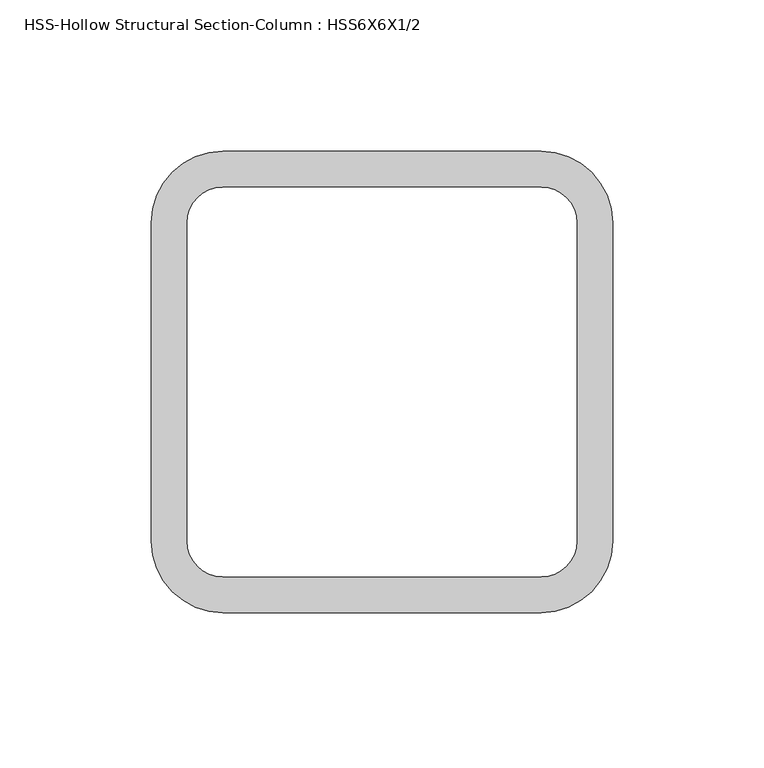
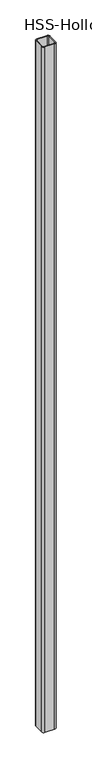
"""IFC4 building model written with IfcOpenShell, lengths in millimetres: column geometry, HSS-Hollow Structural Section-Column : HSS6X6X1/2."""

from ifc_helpers import new_model, si_unit, point, frame, frame_2d, origin, place, context, project, spatial, polyline, circle_curve, trimmed, segment, composite_curve, outline, extrude, source, transform, mapped, element, save


def hss_hollow_structural_section_column_hss6x6x1_2_4c28cf5f(model_context):
    return source(origin(), model_context, "Body", "SweptSolid", [
        extrude(outline(composite_curve([segment(trimmed(circle_curve(frame_2d((52.578, 52.578)), 23.622), [point((52.578, 76.2))], [point((76.2, 52.578))], False, "CARTESIAN"), True, "CONTINUOUS"), segment(polyline([(76.2, 52.578), (76.2, -52.578)]), True, "CONTINUOUS"), segment(trimmed(circle_curve(frame_2d((52.578, -52.578)), 23.622), [point((76.2, -52.578))], [point((52.578, -76.2))], False, "CARTESIAN"), True, "CONTINUOUS"), segment(polyline([(52.578, -76.2), (-52.578, -76.2)]), True, "CONTINUOUS"), segment(trimmed(circle_curve(frame_2d((-52.578, -52.578)), 23.622), [point((-52.578, -76.2))], [point((-76.2, -52.578))], False, "CARTESIAN"), True, "CONTINUOUS"), segment(polyline([(-76.2, -52.578), (-76.2, 52.578)]), True, "CONTINUOUS"), segment(trimmed(circle_curve(frame_2d((-52.578, 52.578)), 23.622), [point((-76.2, 52.578))], [point((-52.578, 76.2))], False, "CARTESIAN"), True, "CONTINUOUS"), segment(polyline([(-52.578, 76.2), (52.578, 76.2)]), True, "CONTINUOUS")], self_intersect=False), holes=[composite_curve([segment(polyline([(52.578, 64.389), (-52.578, 64.389)]), True, "CONTINUOUS"), segment(trimmed(circle_curve(frame_2d((-52.578, 52.578)), 11.811), [point((-52.578, 64.389))], [point((-64.389, 52.578))], True, "CARTESIAN"), True, "CONTINUOUS"), segment(polyline([(-64.389, 52.578), (-64.389, -52.578)]), True, "CONTINUOUS"), segment(trimmed(circle_curve(frame_2d((-52.578, -52.578)), 11.811), [point((-64.389, -52.578))], [point((-52.578, -64.389))], True, "CARTESIAN"), True, "CONTINUOUS"), segment(polyline([(-52.578, -64.389), (52.578, -64.389)]), True, "CONTINUOUS"), segment(trimmed(circle_curve(frame_2d((52.578, -52.578)), 11.811), [point((52.578, -64.389))], [point((64.389, -52.578))], True, "CARTESIAN"), True, "CONTINUOUS"), segment(polyline([(64.389, -52.578), (64.389, 52.578)]), True, "CONTINUOUS"), segment(trimmed(circle_curve(frame_2d((52.578, 52.578)), 11.811), [point((64.389, 52.578))], [point((52.578, 64.389))], True, "CARTESIAN"), True, "CONTINUOUS")], self_intersect=False)]), frame((0.0, 0.0, 4267.2), z_axis=(0.0, 0.0, 1.0), x_axis=(1.0, 0.0, 0.0)), (0.0, 0.0, 1.0), 7823.2),
    ])


if __name__ == "__main__":
    model = new_model("IFC4")
    model_context = context("Model", 3, world=origin())
    ifc_project = project(units=[si_unit("LENGTHUNIT", "METRE", prefix="MILLI")], contexts=[model_context])
    site = spatial("IfcSite", under=ifc_project)
    building = spatial("IfcBuilding", under=site)
    placement = place(None, origin())
    hss_hollow_structural_section_column_hss6x6x1_2_shape = hss_hollow_structural_section_column_hss6x6x1_2_4c28cf5f(model_context)
    element("IfcColumn", 1, ObjectType="HSS-Hollow Structural Section-Column : HSS6X6X1/2", at=placement, inside=building, context=model_context, shape_type="MappedRepresentation", body=[
        mapped(hss_hollow_structural_section_column_hss6x6x1_2_shape, transform((0.0, 0.0, 0.0), x_axis=(1.0, 0.0, 0.0), y_axis=(0.0, 1.0, 0.0), z_axis=(0.0, 0.0, 1.0))),
    ])
    save(model, "model.ifc")

# Revit data of these elements
# Type "HSS-Hollow Structural Section-Column : HSS6X6X1/2"
#   Assembly Code = "B10"
#   Shape = "Square"
#   W = 35.1
#   Ht = 0' - 6"
#   b = 0' - 6"
#   kr = 0' - 0.93"
#   t = 0' - 0.465"
#   A = 0.0676389 SF
#   Structural Material [instance default] = Steel ASTM A500, Grade B, Rectangular and Square
# Element 1 (IfcColumn, "HSS-Hollow Structural Section-Column : HSS6X6X1/2")
#   Materials on its faces: "Steel ASTM A500, Grade B, Rectangular and Square"
# Materials
#   "Steel ASTM A500, Grade B, Rectangular and Square": class "Metal", colour RGB 199 199 199, transparency 0, Description = "Carbon steel", Cost = 0
